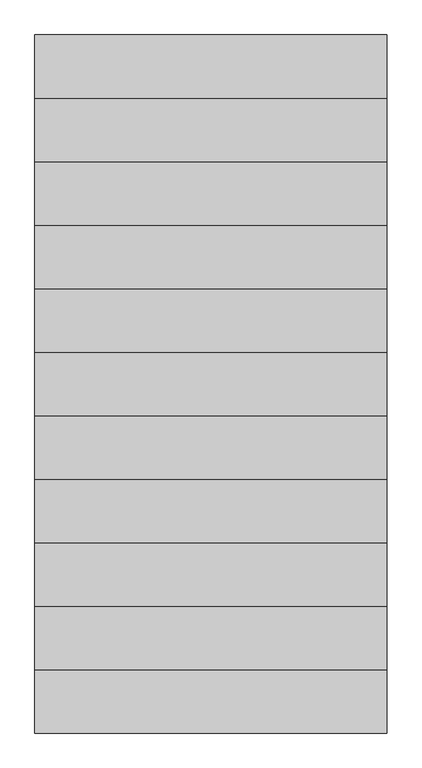
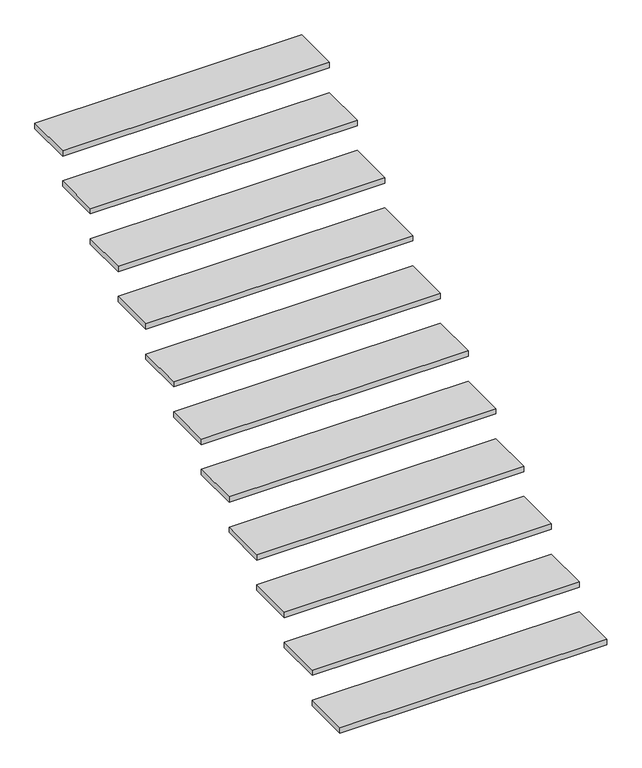
"""IFC4 building model written with IfcOpenShell, lengths in millimetres: stair flight geometry."""

from ifc_helpers import new_model, si_unit, frame, origin, place, context, project, spatial, polyline, outline, extrude, source, transform, mapped, element, save


def stair_flight_650831ce(model_context):
    return source(origin(), model_context, "Body", "SweptSolid", [
        extrude(outline(polyline([(17005.3403387, 2217.6066446), (18505.3403387, 2217.6066446), (18505.3403387, 1947.6066446), (17005.3403387, 1947.6066446), (17005.3403387, 2217.6066446)])), frame((0.0, 0.0, 8028.4395604), z_axis=(0.0, 0.0, 1.0), x_axis=(1.0, 0.0, 0.0)), (0.0, 0.0, 1.0), 32.0),
        extrude(outline(polyline([(17005.3403387, 2487.6066446), (18505.3403387, 2487.6066446), (18505.3403387, 2217.6066446), (17005.3403387, 2217.6066446), (17005.3403387, 2487.6066446)])), frame((0.0, 0.0, 8207.5604396), z_axis=(0.0, 0.0, 1.0), x_axis=(1.0, 0.0, 0.0)), (0.0, 0.0, 1.0), 32.0),
        extrude(outline(polyline([(17005.3403387, 2757.6066446), (18505.3403387, 2757.6066446), (18505.3403387, 2487.6066446), (17005.3403387, 2487.6066446), (17005.3403387, 2757.6066446)])), frame((0.0, 0.0, 8386.6813187), z_axis=(0.0, 0.0, 1.0), x_axis=(1.0, 0.0, 0.0)), (0.0, 0.0, 1.0), 32.0),
        extrude(outline(polyline([(17005.3403387, 3027.6066446), (18505.3403387, 3027.6066446), (18505.3403387, 2757.6066446), (17005.3403387, 2757.6066446), (17005.3403387, 3027.6066446)])), frame((0.0, 0.0, 8565.8021978), z_axis=(0.0, 0.0, 1.0), x_axis=(1.0, 0.0, 0.0)), (0.0, 0.0, 1.0), 32.0),
        extrude(outline(polyline([(17005.3403387, 3297.6066446), (18505.3403387, 3297.6066446), (18505.3403387, 3027.6066446), (17005.3403387, 3027.6066446), (17005.3403387, 3297.6066446)])), frame((0.0, 0.0, 8744.9230769), z_axis=(0.0, 0.0, 1.0), x_axis=(1.0, 0.0, 0.0)), (0.0, 0.0, 1.0), 32.0),
        extrude(outline(polyline([(17005.3403387, 3567.6066446), (18505.3403387, 3567.6066446), (18505.3403387, 3297.6066446), (17005.3403387, 3297.6066446), (17005.3403387, 3567.6066446)])), frame((0.0, 0.0, 8924.043956), z_axis=(0.0, 0.0, 1.0), x_axis=(1.0, 0.0, 0.0)), (0.0, 0.0, 1.0), 32.0),
        extrude(outline(polyline([(17005.3403387, 3837.6066446), (18505.3403387, 3837.6066446), (18505.3403387, 3567.6066446), (17005.3403387, 3567.6066446), (17005.3403387, 3837.6066446)])), frame((0.0, 0.0, 9103.1648352), z_axis=(0.0, 0.0, 1.0), x_axis=(1.0, 0.0, 0.0)), (0.0, 0.0, 1.0), 32.0),
        extrude(outline(polyline([(17005.3403387, 4107.6066446), (18505.3403387, 4107.6066446), (18505.3403387, 3837.6066446), (17005.3403387, 3837.6066446), (17005.3403387, 4107.6066446)])), frame((0.0, 0.0, 9282.2857143), z_axis=(0.0, 0.0, 1.0), x_axis=(1.0, 0.0, 0.0)), (0.0, 0.0, 1.0), 32.0),
        extrude(outline(polyline([(17005.3403387, 4377.6066446), (18505.3403387, 4377.6066446), (18505.3403387, 4107.6066446), (17005.3403387, 4107.6066446), (17005.3403387, 4377.6066446)])), frame((0.0, 0.0, 9461.4065934), z_axis=(0.0, 0.0, 1.0), x_axis=(1.0, 0.0, 0.0)), (0.0, 0.0, 1.0), 32.0),
        extrude(outline(polyline([(17005.3403387, 4647.6066446), (18505.3403387, 4647.6066446), (18505.3403387, 4377.6066446), (17005.3403387, 4377.6066446), (17005.3403387, 4647.6066446)])), frame((0.0, 0.0, 9640.5274725), z_axis=(0.0, 0.0, 1.0), x_axis=(1.0, 0.0, 0.0)), (0.0, 0.0, 1.0), 32.0),
        extrude(outline(polyline([(17005.3403387, 4917.6066446), (18505.3403387, 4917.6066446), (18505.3403387, 4647.6066446), (17005.3403387, 4647.6066446), (17005.3403387, 4917.6066446)])), frame((0.0, 0.0, 9819.6483516), z_axis=(0.0, 0.0, 1.0), x_axis=(1.0, 0.0, 0.0)), (0.0, 0.0, 1.0), 32.0),
    ])


if __name__ == "__main__":
    model = new_model("IFC4")
    model_context = context("Model", 3, world=origin())
    ifc_project = project(units=[si_unit("LENGTHUNIT", "METRE", prefix="MILLI")], contexts=[model_context])
    site = spatial("IfcSite", under=ifc_project)
    building = spatial("IfcBuilding", under=site)
    placement = place(None, origin())
    stair_flight_shape = stair_flight_650831ce(model_context)
    element("IfcStairFlight", 1, at=placement, inside=building, context=model_context, shape_type="MappedRepresentation", body=[
        mapped(stair_flight_shape, transform((0.0, 0.0, 0.0), x_axis=(1.0, 0.0, 0.0), y_axis=(0.0, 1.0, 0.0), z_axis=(0.0, 0.0, 1.0))),
    ])
    save(model, "model.ifc")

# Revit data of these elements
# Element 1 (IfcStairFlight)
#   Materials on its faces: "철강"
# Materials
#   "철강": class "Generic", colour RGB 143 142 141, transparency 0, Description = "철골+가공조립+세우기", Cost = 0
